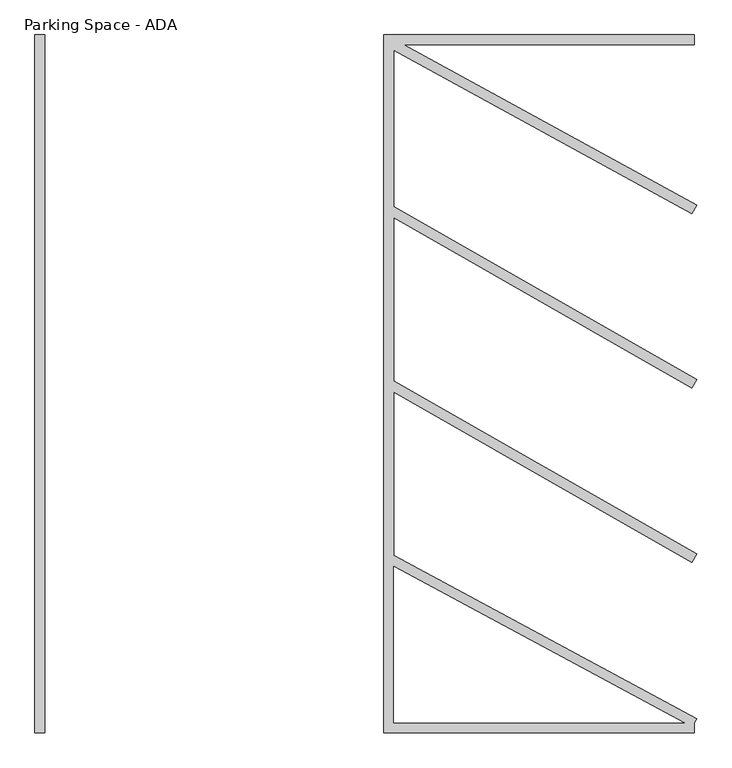
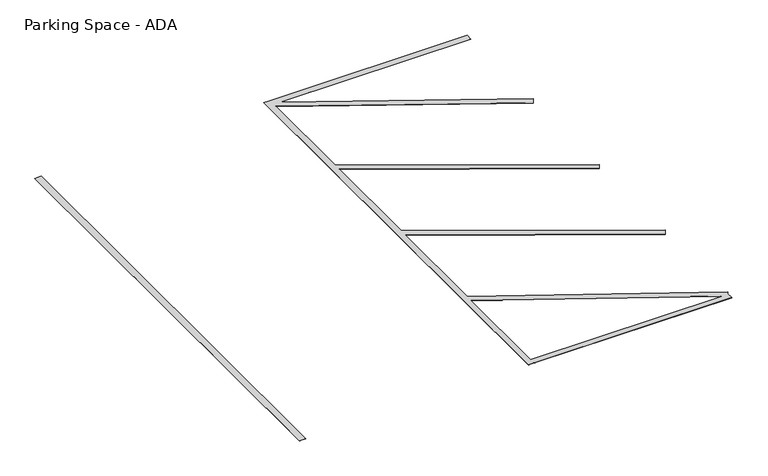
"""IFC4 building model written with IfcOpenShell, lengths in millimetres: proxy geometry, Parking Space - ADA : 9' x 18' (8' Aisle)."""

from ifc_helpers import new_model, si_unit, origin, origin_with_axes, place, context, project, spatial, polyline, outline, extrude, source, transform, mapped, element, save


def parking_space_ada_2abbe88e(model_context):
    return source(origin(), model_context, "Body", "SweptSolid", [
        extrude(outline(polyline([(4046.2620479, -859.2253385), (3970.0620479, -859.2253385), (3970.0620479, 4627.1746615), (4046.2620479, 4627.1746615), (6408.4620479, 4627.1746615), (6408.4620479, 4550.9746615), (4125.4996019, 4550.9746615), (6426.7817704, 3288.9812143), (6390.1423254, 3222.1681088), (4046.2620479, 4507.5218093), (4046.2620479, 3277.6849501), (6427.3649414, 1917.0547253), (6389.5591543, 1850.8945978), (4046.2620479, 3189.9215158), (4046.2620479, 1906.0849501), (6427.3649414, 545.4547253), (6389.5591543, 479.2945978), (4046.2620479, 1818.3215158), (4046.2620479, 535.1071205), (6426.55698, -749.4964937), (6408.4620479, -783.0253385), (6408.4620479, -859.2253385), (4046.2620479, -859.2253385)]), holes=[polyline([(6328.2401387, -783.0253385), (4046.2620479, 448.5183931), (4046.2620479, -783.0253385), (6328.2401387, -783.0253385)])]), origin_with_axes(), (0.0, 0.0, 1.0), 1.5875),
        extrude(outline(polyline([(1303.0620479, -859.2253385), (1226.8620479, -859.2253385), (1226.8620479, 4627.1746615), (1303.0620479, 4627.1746615), (1303.0620479, -859.2253385)])), origin_with_axes(), (0.0, 0.0, 1.0), 1.5875),
    ])


if __name__ == "__main__":
    model = new_model("IFC4")
    model_context = context("Model", 3, world=origin())
    ifc_project = project(units=[si_unit("LENGTHUNIT", "METRE", prefix="MILLI")], contexts=[model_context])
    site = spatial("IfcSite", under=ifc_project)
    building = spatial("IfcBuilding", under=site)
    placement = place(None, origin())
    parking_space_ada_shape = parking_space_ada_2abbe88e(model_context)
    element("IfcBuildingElementProxy", 1, Name="Parking Space - ADA : 9' x 18' (8' Aisle)", ObjectType="Parking Space - ADA : 9' x 18' (8' Aisle)", at=placement, inside=building, context=model_context, shape_type="MappedRepresentation", body=[
        mapped(parking_space_ada_shape, transform((0.0, 0.0, 0.0), x_axis=(1.0, 0.0, 0.0), y_axis=(0.0, 1.0, 0.0), z_axis=(0.0, 0.0, 1.0))),
    ])
    save(model, "model.ifc")

# Revit data of these elements
# Type "Parking Space - ADA : 9' x 18' (8' Aisle)"
#   Accesible Aisle = 2438.4 mm
#   Length = 5486.4 mm
#   Width = 2743.2 mm
# Element 1 (IfcBuildingElementProxy, "Parking Space - ADA : 9' x 18' (8' Aisle)")
#   Materials on its faces: "Parking Stripe"
# Materials
#   "Parking Stripe": class "Paint", colour RGB 250 250 91, transparency 0, Cost = 0
